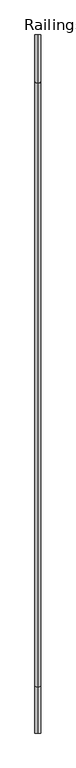
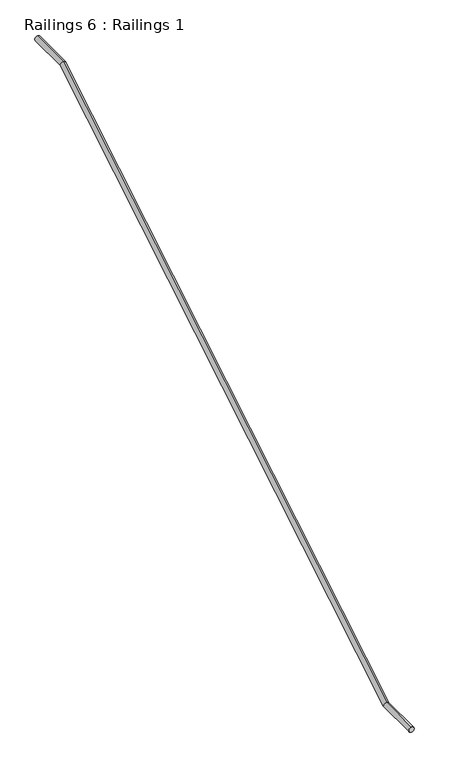
"""IFC4 building model written with IfcOpenShell, lengths in millimetres: railing geometry, Railings 6 : Railings 1."""

from ifc_helpers import new_model, si_unit, frame, origin, place, context, project, spatial, circle_curve, ellipse_curve, source, transform, mapped, element, save
from ifc_brep_helpers import plane_surface, cylinder_surface, advanced_brep


def railings_6_railings_1_e01e9050(model_context):
    return source(origin(), model_context, "Body", "AdvancedBrep", [
        advanced_brep(
        [(32273.1661999, 34864.3618167, 267230.225), (32273.1661999, 34864.3618167, 267268.325), (32273.1661999, 30343.1618167, 264874.375), (32273.1661999, 30343.1618167, 264912.475), (32273.1661999, 34564.8554866, 267230.225), (32273.1661999, 34554.2681467, 267268.325), (32273.1661999, 30653.2554866, 264874.375), (32273.1661999, 30642.6681467, 264912.475)],
        [
            (0, 1, circle_curve(frame((32273.1661999, 34864.3618167, 267249.275), z_axis=(0.0, 1.0, 0.0), x_axis=(0.0, 0.0, 1.0)), 19.05)),
            (1, 0, circle_curve(frame((32273.1661999, 34864.3618167, 267249.275), z_axis=(0.0, 1.0, 0.0), x_axis=(0.0, 0.0, 1.0)), 19.05)),
            (2, 3, circle_curve(frame((32273.1661999, 30343.1618167, 264893.425), z_axis=(0.0, -1.0, 0.0), x_axis=(0.0, 0.0, 1.0)), 19.05)),
            (3, 2, circle_curve(frame((32273.1661999, 30343.1618167, 264893.425), z_axis=(0.0, -1.0, 0.0), x_axis=(0.0, 0.0, 1.0)), 19.05)),
            (0, 4),
            (4, 5, ellipse_curve(frame((32273.1661999, 34559.5618167, 267249.275), z_axis=(0.0, 0.9634917766912388, 0.2677379245612399), x_axis=(0.0, 0.2677379245612395, -0.9634917766912388)), 19.7718346, 19.05)),
            (5, 1),
            (5, 4, ellipse_curve(frame((32273.1661999, 34559.5618167, 267249.275), z_axis=(0.0, 0.9634917766912388, 0.2677379245612399), x_axis=(0.0, 0.2677379245612395, -0.9634917766912388)), 19.7718346, 19.05)),
            (4, 6),
            (6, 7, ellipse_curve(frame((32273.1661999, 30647.9618167, 264893.425), z_axis=(0.0, 0.9634917766912388, 0.2677379245612399), x_axis=(0.0, -0.26773792456124046, 0.9634917766912386)), 19.7718346, 19.05)),
            (7, 5),
            (7, 6, ellipse_curve(frame((32273.1661999, 30647.9618167, 264893.425), z_axis=(0.0, 0.9634917766912388, 0.2677379245612399), x_axis=(0.0, -0.26773792456124046, 0.9634917766912386)), 19.7718346, 19.05)),
            (6, 2),
            (3, 7),
        ],
        [
            plane_surface(frame((32292.2161999, 34864.3618167, 267249.275), z_axis=(0.0, 1.0, 0.0), x_axis=(1.0, 0.0, 0.0))),
            plane_surface(frame((32292.2161999, 30343.1618167, 264893.425), z_axis=(0.0, -1.0, 0.0), x_axis=(1.0, 0.0, 0.0))),
            cylinder_surface(frame((32273.1661999, 34864.3618167, 267249.275), z_axis=(0.0, 1.0, 0.0), x_axis=(0.0, 0.0, 1.0)), 19.05),
            cylinder_surface(frame((32273.1661999, 34559.5618167, 267249.275), z_axis=(0.0, 0.8566328075032797, 0.5159265772462676), x_axis=(0.0, -0.5159265772462676, 0.8566328075032797)), 19.05),
            cylinder_surface(frame((32273.1661999, 30647.9618167, 264893.425), z_axis=(0.0, 1.0, 0.0), x_axis=(0.0, 0.0, 1.0)), 19.05),
        ],
        [
            (0, [[1, 2]]),
            (1, [[3, 4]]),
            (2, [[-1, 5, 6, 7]]),
            (2, [[-2, -7, 8, -5]]),
            (3, [[-6, 9, 10, 11]]),
            (3, [[-8, -11, 12, -9]]),
            (4, [[-10, 13, -4, 14]]),
            (4, [[-12, -14, -3, -13]]),
        ],
    ),
    ])


if __name__ == "__main__":
    model = new_model("IFC4")
    model_context = context("Model", 3, world=origin())
    ifc_project = project(units=[si_unit("LENGTHUNIT", "METRE", prefix="MILLI")], contexts=[model_context])
    site = spatial("IfcSite", under=ifc_project)
    building = spatial("IfcBuilding", under=site)
    placement = place(None, origin())
    railings_6_railings_1_shape = railings_6_railings_1_e01e9050(model_context)
    element("IfcRailing", 1, ObjectType="Railings 6 : Railings 1", at=placement, inside=building, context=model_context, shape_type="MappedRepresentation", body=[
        mapped(railings_6_railings_1_shape, transform((0.0, 0.0, 0.0), x_axis=(1.0, 0.0, 0.0), y_axis=(0.0, 1.0, 0.0), z_axis=(0.0, 0.0, 1.0))),
    ])
    save(model, "model.ifc")

# Revit data of these elements
# Element 1 (IfcRailing, "Railings 6 : Railings 1")
#   Materials on its faces: "ALUM. RAILING"
# Materials
#   "ALUM. RAILING": class "Generic", colour RGB 255 255 255, transparency 0, Cost = 0
